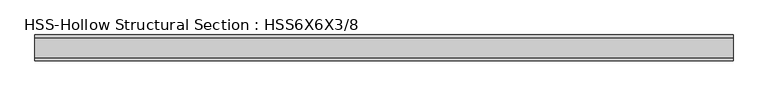
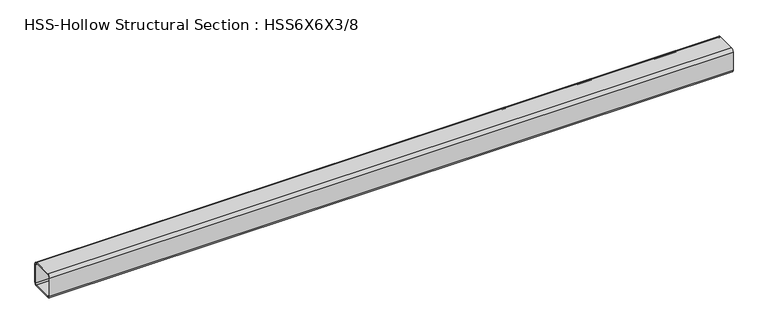
"""IFC4 building model written with IfcOpenShell, lengths in millimetres: member geometry, HSS-Hollow Structural Section : HSS6X6X3/8."""

from ifc_helpers import new_model, si_unit, point, frame, frame_2d, origin, place, context, project, spatial, polyline, circle_curve, trimmed, segment, composite_curve, outline, extrude, source, transform, mapped, element, save


def hss_hollow_structural_section_hss6x6x3_8_cecd57c8(model_context):
    return source(origin(), model_context, "Body", "SweptSolid", [
        extrude(outline(composite_curve([segment(polyline([(76.2, 58.4708), (76.2, -58.4708)]), True, "CONTINUOUS"), segment(trimmed(circle_curve(frame_2d((58.4708, -58.4708)), 17.7292), [point((76.2, -58.4708))], [point((58.4708, -76.2))], False, "CARTESIAN"), True, "CONTINUOUS"), segment(polyline([(58.4708, -76.2), (-58.4708, -76.2)]), True, "CONTINUOUS"), segment(trimmed(circle_curve(frame_2d((-58.4708, -58.4708)), 17.7292), [point((-58.4708, -76.2))], [point((-76.2, -58.4708))], False, "CARTESIAN"), True, "CONTINUOUS"), segment(polyline([(-76.2, -58.4708), (-76.2, 58.4708)]), True, "CONTINUOUS"), segment(trimmed(circle_curve(frame_2d((-58.4708, 58.4708)), 17.7292), [point((-76.2, 58.4708))], [point((-58.4708, 76.2))], False, "CARTESIAN"), True, "CONTINUOUS"), segment(polyline([(-58.4708, 76.2), (58.4708, 76.2)]), True, "CONTINUOUS"), segment(trimmed(circle_curve(frame_2d((58.4708, 58.4708)), 17.7292), [point((58.4708, 76.2))], [point((76.2, 58.4708))], False, "CARTESIAN"), True, "CONTINUOUS")], self_intersect=False), holes=[composite_curve([segment(trimmed(circle_curve(frame_2d((-58.4708, 58.4708)), 8.8646), [point((-58.4708, 67.3354))], [point((-67.3354, 58.4708))], True, "CARTESIAN"), True, "CONTINUOUS"), segment(polyline([(-67.3354, 58.4708), (-67.3354, -58.4708)]), True, "CONTINUOUS"), segment(trimmed(circle_curve(frame_2d((-58.4708, -58.4708)), 8.8646), [point((-67.3354, -58.4708))], [point((-58.4708, -67.3354))], True, "CARTESIAN"), True, "CONTINUOUS"), segment(polyline([(-58.4708, -67.3354), (58.4708, -67.3354)]), True, "CONTINUOUS"), segment(trimmed(circle_curve(frame_2d((58.4708, -58.4708)), 8.8646), [point((58.4708, -67.3354))], [point((67.3354, -58.4708))], True, "CARTESIAN"), True, "CONTINUOUS"), segment(polyline([(67.3354, -58.4708), (67.3354, 58.4708)]), True, "CONTINUOUS"), segment(trimmed(circle_curve(frame_2d((58.4708, 58.4708)), 8.8646), [point((67.3354, 58.4708))], [point((58.4708, 67.3354))], True, "CARTESIAN"), True, "CONTINUOUS"), segment(polyline([(58.4708, 67.3354), (-58.4708, 67.3354)]), True, "CONTINUOUS")], self_intersect=False)]), frame((-2040.8268892, 0.0, 0.0), z_axis=(1.0, 0.0, 0.0), x_axis=(0.0, 1.0, 0.0)), (0.0, 0.0, 1.0), 4142.4003489),
    ])


if __name__ == "__main__":
    model = new_model("IFC4")
    model_context = context("Model", 3, world=origin())
    ifc_project = project(units=[si_unit("LENGTHUNIT", "METRE", prefix="MILLI")], contexts=[model_context])
    site = spatial("IfcSite", under=ifc_project)
    building = spatial("IfcBuilding", under=site)
    placement = place(None, origin())
    hss_hollow_structural_section_hss6x6x3_8_shape = hss_hollow_structural_section_hss6x6x3_8_cecd57c8(model_context)
    element("IfcMember", 1, ObjectType="HSS-Hollow Structural Section : HSS6X6X3/8", at=placement, inside=building, context=model_context, shape_type="MappedRepresentation", body=[
        mapped(hss_hollow_structural_section_hss6x6x3_8_shape, transform((0.0, 0.0, 0.0), x_axis=(1.0, 0.0, 0.0), y_axis=(0.0, 1.0, 0.0), z_axis=(0.0, 0.0, 1.0))),
    ])
    save(model, "model.ifc")

# Revit data of these elements
# Type "HSS-Hollow Structural Section : HSS6X6X3/8"
#   Assembly Code = "B10"
#   Shape = "Square"
#   W = 27.4
#   Ht = 0' - 6"
#   Length [instance default] = 5' - 0"
#   b = 0' - 6"
#   kr = 0' - 0.698"
#   t = 0' - 0.349"
#   A = 0.0526389 SF
#   Structural Material [instance default] = Steel ASTM A500, Grade B, Rectangular and Square
# Element 1 (IfcMember, "HSS-Hollow Structural Section : HSS6X6X3/8")
#   Materials on its faces: "Steel ASTM A500, Grade B, Rectangular and Square"
# Materials
#   "Steel ASTM A500, Grade B, Rectangular and Square": class "Metal", colour RGB 199 199 199, transparency 0, Description = "Carbon steel", Cost = 0
